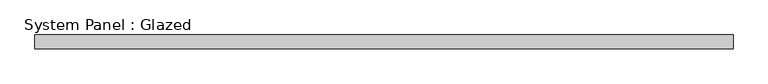
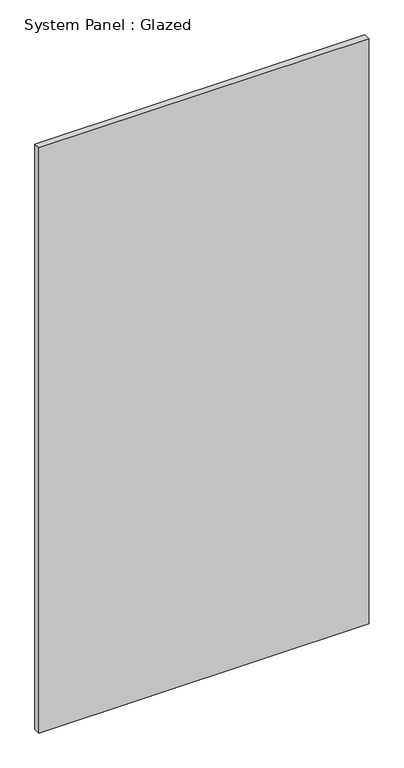
"""IFC4 building model written with IfcOpenShell, lengths in millimetres: plate geometry, System Panel : Glazed."""

from ifc_helpers import new_model, si_unit, origin, origin_with_axes, place, context, project, spatial, polyline, outline, extrude, source, transform, mapped, element, save


def system_panel_glazed_eec4e8b3(model_context):
    return source(origin(), model_context, "Body", "SweptSolid", [
        extrude(outline(polyline([(626.7857144, 24.5), (-626.7857144, 24.5), (-626.7857144, 49.5), (626.7857144, 49.5), (626.7857144, 24.5)])), origin_with_axes(), (0.0, 0.0, 1.0), 2350.0),
    ])


if __name__ == "__main__":
    model = new_model("IFC4")
    model_context = context("Model", 3, world=origin())
    ifc_project = project(units=[si_unit("LENGTHUNIT", "METRE", prefix="MILLI")], contexts=[model_context])
    site = spatial("IfcSite", under=ifc_project)
    building = spatial("IfcBuilding", under=site)
    placement = place(None, origin())
    system_panel_glazed_shape = system_panel_glazed_eec4e8b3(model_context)
    element("IfcPlate", 1, ObjectType="System Panel : Glazed", at=placement, inside=building, context=model_context, shape_type="MappedRepresentation", body=[
        mapped(system_panel_glazed_shape, transform((0.0, 0.0, 0.0), x_axis=(1.0, 0.0, 0.0), y_axis=(0.0, 1.0, 0.0), z_axis=(0.0, 0.0, 1.0))),
    ])
    save(model, "model.ifc")

# Revit data of these elements
# Type "System Panel : Glazed"
#   Construction Type Id = "GSP4R"
#   Analytic Construction = "1/8 in Pilkington single glazing"
#   Visual Light Transmittance = 0.9
#   Solar Heat Gain Coefficient = 0.86
#   Heat Transfer Coefficient (U) = 6.7069 W/(m²·K)
#   Define Thermal Properties by = 1
# Element 1 (IfcPlate, "System Panel : Glazed")
#   Materials on its faces: "Glass"
# Materials
#   "Glass": class "Glass", colour RGB 0 128 192, transparency 0.75, Description = "Soda Lime Glass", Cost = 0
